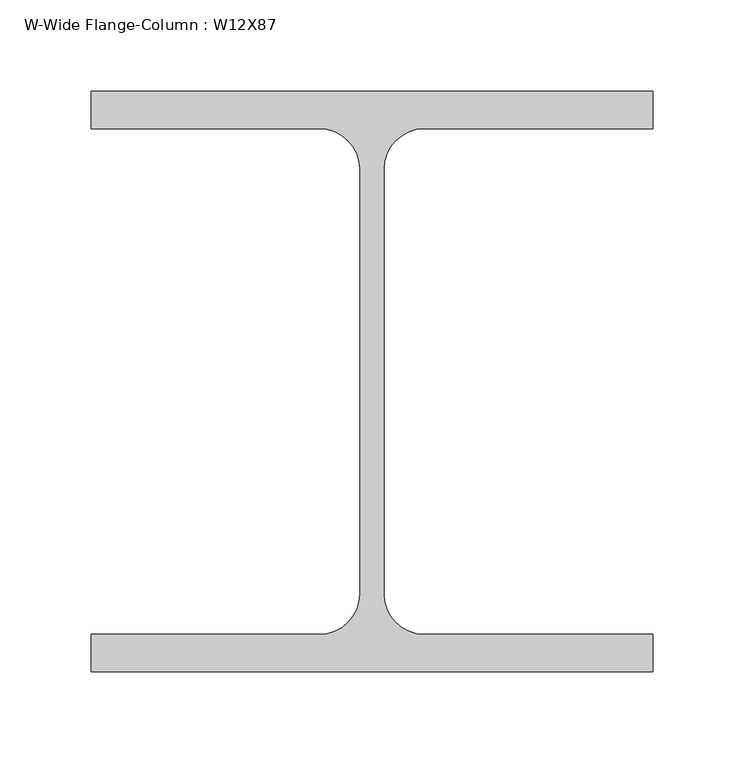
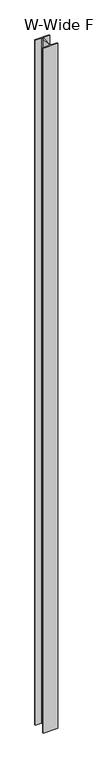
"""IFC4 building model written with IfcOpenShell, lengths in millimetres: column geometry, W-Wide Flange-Column : W12X87."""

from ifc_helpers import new_model, si_unit, point, frame, frame_2d, origin, place, context, project, spatial, polyline, circle_curve, trimmed, segment, composite_curve, outline, extrude, source, transform, mapped, element, save


def w_wide_flange_column_w12x87_da20b1fb(model_context):
    return source(origin(), model_context, "Body", "SweptSolid", [
        extrude(outline(composite_curve([segment(polyline([(153.9875, 159.146875), (153.9875, 138.6085937), (28.8726562, 138.6085937)]), True, "CONTINUOUS"), segment(trimmed(circle_curve(frame_2d((28.8726562, 116.284375)), 22.3242188), [point((28.8726562, 138.6085937))], [point((6.5484375, 116.284375))], True, "CARTESIAN"), True, "CONTINUOUS"), segment(polyline([(6.5484375, 116.284375), (6.5484375, -116.284375)]), True, "CONTINUOUS"), segment(trimmed(circle_curve(frame_2d((28.8726562, -116.284375)), 22.3242188), [point((6.5484375, -116.284375))], [point((28.8726562, -138.6085937))], True, "CARTESIAN"), True, "CONTINUOUS"), segment(polyline([(28.8726562, -138.6085937), (153.9875, -138.6085937), (153.9875, -159.146875), (-153.9875, -159.146875), (-153.9875, -138.6085937), (-28.8726563, -138.6085937)]), True, "CONTINUOUS"), segment(trimmed(circle_curve(frame_2d((-28.8726563, -116.284375)), 22.3242188), [point((-28.8726563, -138.6085937))], [point((-6.5484375, -116.284375))], True, "CARTESIAN"), True, "CONTINUOUS"), segment(polyline([(-6.5484375, -116.284375), (-6.5484375, 116.284375)]), True, "CONTINUOUS"), segment(trimmed(circle_curve(frame_2d((-28.8726563, 116.284375)), 22.3242188), [point((-6.5484375, 116.284375))], [point((-28.8726563, 138.6085937))], True, "CARTESIAN"), True, "CONTINUOUS"), segment(polyline([(-28.8726563, 138.6085937), (-153.9875, 138.6085937), (-153.9875, 159.146875), (153.9875, 159.146875)]), True, "CONTINUOUS")], self_intersect=False)), frame((0.0, 0.0, -914.4), z_axis=(0.0, 0.0, 1.0), x_axis=(1.0, 0.0, 0.0)), (0.0, 0.0, 1.0), 15544.8),
    ])


if __name__ == "__main__":
    model = new_model("IFC4")
    model_context = context("Model", 3, world=origin())
    ifc_project = project(units=[si_unit("LENGTHUNIT", "METRE", prefix="MILLI")], contexts=[model_context])
    site = spatial("IfcSite", under=ifc_project)
    building = spatial("IfcBuilding", under=site)
    placement = place(None, origin())
    w_wide_flange_column_w12x87_shape = w_wide_flange_column_w12x87_da20b1fb(model_context)
    element("IfcColumn", 1, ObjectType="W-Wide Flange-Column : W12X87", at=placement, inside=building, context=model_context, shape_type="MappedRepresentation", body=[
        mapped(w_wide_flange_column_w12x87_shape, transform((0.0, 0.0, 0.0), x_axis=(1.0, 0.0, 0.0), y_axis=(0.0, 1.0, 0.0), z_axis=(0.0, 0.0, 1.0))),
    ])
    save(model, "model.ifc")

# Revit data of these elements
# Type "W-Wide Flange-Column : W12X87"
#   Assembly Code = "B10"
#   A = 0.18 SF
#   W = 87
#   bf = 1' - 0 1/8"
#   d = 1' - 0 17/32"
#   k = 0' - 1 11/16"
#   kr = 0' - 0 225/256"
#   tf = 0' - 0 207/256"
#   tw = 0' - 0 33/64"
#   Structural Material [instance default] = Metal - Steel - ASTM A992
# Element 1 (IfcColumn, "W-Wide Flange-Column : W12X87")
#   Materials on its faces: "Metal - Steel - ASTM A992"
# Materials
#   "Metal - Steel - ASTM A992": class "Unassigned", colour RGB 199 199 199, transparency 0, Description = "Steel ASTM A992"
